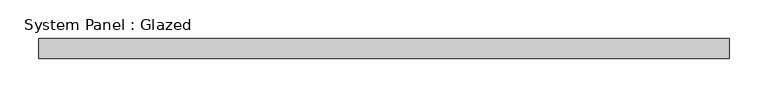
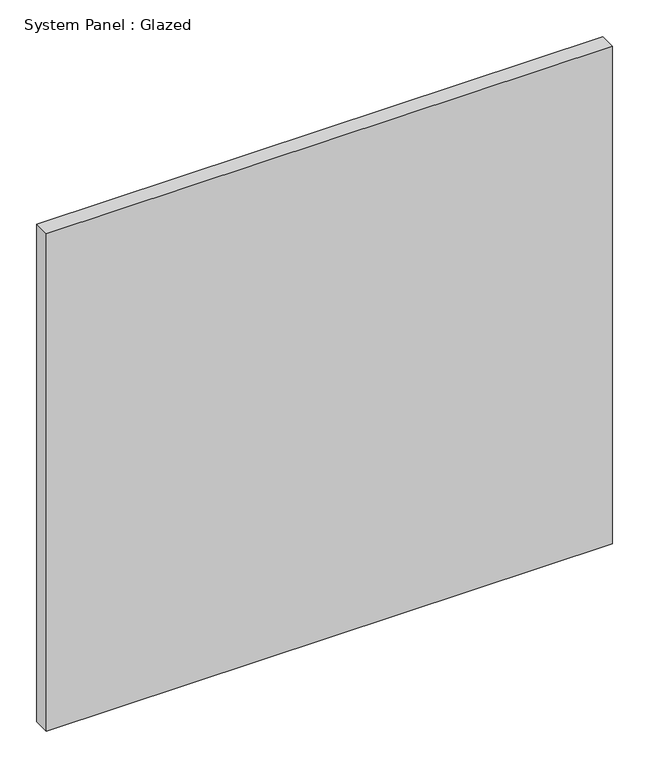
"""IFC4 building model written with IfcOpenShell, lengths in millimetres: plate geometry, System Panel : Glazed."""

from ifc_helpers import new_model, si_unit, origin, origin_with_axes, place, context, project, spatial, polyline, outline, extrude, source, transform, mapped, element, save


def system_panel_glazed_f362540c(model_context):
    return source(origin(), model_context, "Body", "SweptSolid", [
        extrude(outline(polyline([(444.4999998, -44.45), (-444.4999998, -44.45), (-444.4999998, -19.05), (444.4999998, -19.05), (444.4999998, -44.45)])), origin_with_axes(), (0.0, 0.0, 1.0), 825.5),
    ])


if __name__ == "__main__":
    model = new_model("IFC4")
    model_context = context("Model", 3, world=origin())
    ifc_project = project(units=[si_unit("LENGTHUNIT", "METRE", prefix="MILLI")], contexts=[model_context])
    site = spatial("IfcSite", under=ifc_project)
    building = spatial("IfcBuilding", under=site)
    placement = place(None, origin())
    system_panel_glazed_shape = system_panel_glazed_f362540c(model_context)
    element("IfcPlate", 1, ObjectType="System Panel : Glazed", at=placement, inside=building, context=model_context, shape_type="MappedRepresentation", body=[
        mapped(system_panel_glazed_shape, transform((0.0, 0.0, 0.0), x_axis=(1.0, 0.0, 0.0), y_axis=(0.0, 1.0, 0.0), z_axis=(0.0, 0.0, 1.0))),
    ])
    save(model, "model.ifc")

# Revit data of these elements
# Element 1 (IfcPlate, "System Panel : Glazed")
#   Materials on its faces: "Glass"
# Materials
#   "Glass": class "Glass", colour RGB 0 128 192, transparency 0.75
